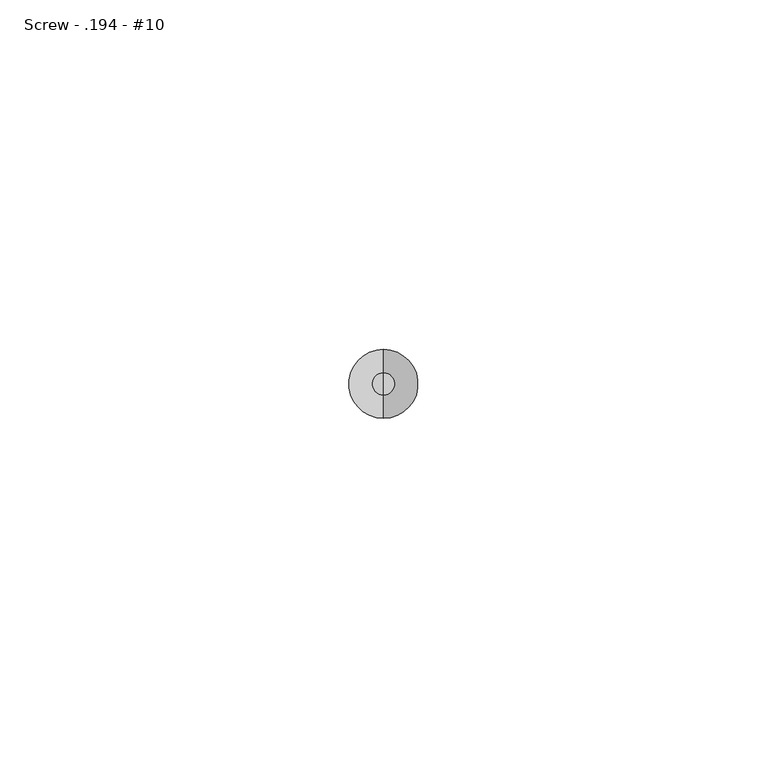
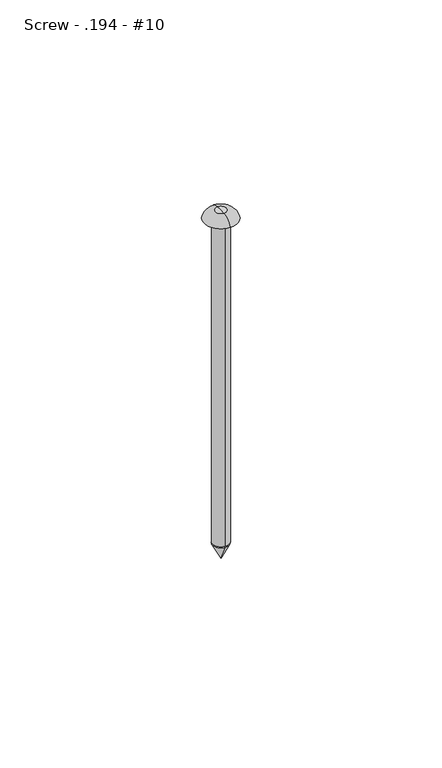
"""IFC4 building model written with IfcOpenShell, lengths in millimetres: fastener geometry, 060523 - W_P_C - Fastenings - Generic : Screw - .194 - #10."""

import ifcopenshell
import ifcopenshell.guid

model = None  # the IFC model being written
_history = None  # IfcOwnerHistory: only IFC2X3 demands one
_inside = {}  # id of a spatial element -> (the spatial element, [elements in it])
_under = {}  # id of a project, library or spatial element -> (it, [spatial elements below it])
_declared = {}  # id of a project -> (the project, [libraries it declares])
_typed = {}  # id of a type object -> (the type object, [elements of that type])
_made_of = {}  # id of a material, layer set ... -> (it, [elements and type objects made of it])


def new_model(schema):
    """Start an empty IFC model of exactly this schema.

    Asked for "IFC4X3", IfcOpenShell would pick the latest addendum, in which some entities
    have other attributes; the version numbers below select the first issue.
    IFC2X3 requires an IfcOwnerHistory on every rooted entity: one is made here for all.
    """
    global model, _history
    if schema == "IFC4X3":
        model = ifcopenshell.file(schema_version=(4, 3, 0, 0))
    else:
        model = ifcopenshell.file(schema=schema)
    _inside.clear()
    _under.clear()
    _declared.clear()
    _typed.clear()
    _made_of.clear()
    _history = None
    if model.schema == "IFC2X3":
        org = make("IfcOrganization", Name="unknown")
        user = make(
            "IfcPersonAndOrganization",
            ThePerson=make("IfcPerson", FamilyName="unknown"),
            TheOrganization=org,
        )
        app = make(
            "IfcApplication",
            ApplicationDeveloper=org,
            Version="unknown",
            ApplicationFullName="unknown",
            ApplicationIdentifier="unknown",
        )
        _history = make(
            "IfcOwnerHistory",
            OwningUser=user,
            OwningApplication=app,
            ChangeAction="ADDED",
            CreationDate=0,
        )
    return model


def make(cls, **values):
    """One entity of the class cls with the attributes given. An attribute that is None is left unset."""
    return model.create_entity(
        cls, **{name: value for name, value in values.items() if value is not None}
    )


def rooted(cls, **values):
    """An entity with a GlobalId (a new one), such as an element, a storey or a relation."""
    return make(cls, GlobalId=ifcopenshell.guid.new(), OwnerHistory=_history, **values)


def si_unit(unit_type, name, prefix=None):
    """IfcSIUnit, for example si_unit("LENGTHUNIT", "METRE", prefix="MILLI")."""
    return make("IfcSIUnit", UnitType=unit_type, Prefix=prefix, Name=name)


def assignment(units):
    """IfcUnitAssignment: the units of a project."""
    return None if units is None else make("IfcUnitAssignment", Units=units)


def point(xyz):
    """IfcCartesianPoint."""
    return None if xyz is None else make("IfcCartesianPoint", Coordinates=xyz)


def direction(xyz):
    """IfcDirection."""
    return None if xyz is None else make("IfcDirection", DirectionRatios=xyz)


def frame(location, z_axis=None, x_axis=None):
    """IfcAxis2Placement3D, a coordinate frame: its origin and axes. An axis left out is left unset."""
    return make(
        "IfcAxis2Placement3D",
        Location=point(location),
        Axis=direction(z_axis),
        RefDirection=direction(x_axis),
    )


def frame_2d(location, x_axis=None):
    """IfcAxis2Placement2D, a coordinate frame in the plane: its origin and x axis."""
    return make(
        "IfcAxis2Placement2D", Location=point(location), RefDirection=direction(x_axis)
    )


def origin():
    """The frame at (0, 0, 0) with its axes left unset."""
    return frame((0.0, 0.0, 0.0))


def origin_2d():
    """The frame at (0, 0) in the plane with its x axis left unset."""
    return frame_2d((0.0, 0.0))


def place(relative_to, where):
    """IfcLocalPlacement: puts the frame where relative to a parent placement (None: the world)."""
    return make(
        "IfcLocalPlacement", PlacementRelTo=relative_to, RelativePlacement=where
    )


def context(
    kind, dimensions, precision=None, world=None, true_north=None, identifier=None
):
    """IfcGeometricRepresentationContext, for example the 3D "Model" context."""
    return make(
        "IfcGeometricRepresentationContext",
        ContextIdentifier=identifier,
        ContextType=kind,
        CoordinateSpaceDimension=dimensions,
        Precision=precision,
        WorldCoordinateSystem=world,
        TrueNorth=true_north,
    )


def project(units=None, contexts=None):
    """IfcProject with its units and contexts."""
    return rooted(
        "IfcProject",
        Name="project",
        RepresentationContexts=contexts,
        UnitsInContext=assignment(units),
    )


def spatial(cls, under=None, at=None, **own):
    """A site, building, storey or space (cls), placed at a placement, below another one or the project."""
    s = rooted(cls, ObjectPlacement=at, **own)
    if under is not None:
        _under.setdefault(under.id(), (under, []))[1].append(s)
    return s


def polyline(points):
    """IfcPolyline through the points."""
    return make("IfcPolyline", Points=[point(p) for p in points])


def circle_curve(where, radius):
    """IfcCircle in the frame where."""
    return make("IfcCircle", Position=where, Radius=radius)


def ellipse_curve(where, semi_axis1, semi_axis2):
    """IfcEllipse in the frame where."""
    return make(
        "IfcEllipse", Position=where, SemiAxis1=semi_axis1, SemiAxis2=semi_axis2
    )


def trimmed(basis, trim1, trim2, sense, master):
    """IfcTrimmedCurve: the piece of a basis curve between two trims."""
    return make(
        "IfcTrimmedCurve",
        BasisCurve=basis,
        Trim1=trim1,
        Trim2=trim2,
        SenseAgreement=sense,
        MasterRepresentation=master,
    )


def segment(curve, same_sense, transition):
    """IfcCompositeCurveSegment."""
    return make(
        "IfcCompositeCurveSegment",
        Transition=transition,
        SameSense=same_sense,
        ParentCurve=curve,
    )


def composite_curve(segments, self_intersect=None):
    """IfcCompositeCurve: segments joined end to end."""
    return make("IfcCompositeCurve", Segments=segments, SelfIntersect=self_intersect)


def outline(outer, holes=None, kind="AREA"):
    """IfcArbitraryClosedProfileDef: a profile drawn as a closed curve; with holes, ...WithVoids."""
    if holes is None:
        return make("IfcArbitraryClosedProfileDef", ProfileType=kind, OuterCurve=outer)
    return make(
        "IfcArbitraryProfileDefWithVoids",
        ProfileType=kind,
        OuterCurve=outer,
        InnerCurves=holes,
    )


def extrude(swept, where, along, depth):
    """IfcExtrudedAreaSolid: the profile swept, set in the frame where, extruded along a direction by depth."""
    return make(
        "IfcExtrudedAreaSolid",
        SweptArea=swept,
        Position=where,
        ExtrudedDirection=direction(along),
        Depth=depth,
    )


def shape(context_of_items, identifier, shape_type, items):
    """IfcShapeRepresentation: the items that make up one representation, for example the "Body"."""
    return make(
        "IfcShapeRepresentation",
        ContextOfItems=context_of_items,
        RepresentationIdentifier=identifier,
        RepresentationType=shape_type,
        Items=items,
    )


def source(mapping_origin, context_of_items, identifier, shape_type, items):
    """IfcRepresentationMap: a shape defined once, which mapped items show again and again."""
    return make(
        "IfcRepresentationMap",
        MappingOrigin=mapping_origin,
        MappedRepresentation=shape(context_of_items, identifier, shape_type, items),
    )


def transform(
    local_origin,
    x_axis=None,
    y_axis=None,
    z_axis=None,
    scale=None,
    scale2=None,
    scale3=None,
    uniform=True,
):
    """IfcCartesianTransformationOperator3D, or its non-uniform kind. x_axis, y_axis, z_axis: its Axis1, 2, 3."""
    if uniform:
        return make(
            "IfcCartesianTransformationOperator3D",
            Axis1=direction(x_axis),
            Axis2=direction(y_axis),
            LocalOrigin=point(local_origin),
            Scale=scale,
            Axis3=direction(z_axis),
        )
    return make(
        "IfcCartesianTransformationOperator3DnonUniform",
        Axis1=direction(x_axis),
        Axis2=direction(y_axis),
        LocalOrigin=point(local_origin),
        Scale=scale,
        Axis3=direction(z_axis),
        Scale2=scale2,
        Scale3=scale3,
    )


def mapped(mapping_source, mapping_target):
    """IfcMappedItem: shows the shape of a source again, moved by a transform."""
    return make(
        "IfcMappedItem", MappingSource=mapping_source, MappingTarget=mapping_target
    )


def made_of(thing, what):
    """Note that an element or type object is made of a material, layer set ...; save() writes the relation."""
    if what is not None:
        _made_of.setdefault(what.id(), (what, []))[1].append(thing)
    return thing


def element(
    cls,
    number,
    at=None,
    inside=None,
    cuts=None,
    type_object=None,
    material=None,
    context=None,
    identifier="Body",
    shape_type=None,
    held_by="IfcProductDefinitionShape",
    body=None,
    shapes=None,
    **own,
):
    """One element of the class cls, such as IfcWall. Its Tag is "e" and its number.

    at: its placement. inside: the storey or other place that contains it. cuts: it is an
    opening in that element (IfcRelVoidsElement). A single representation is given by context,
    identifier, shape_type and body (its items); several are given by shapes. held_by: the class
    of the entity that holds the representations. save() writes the other relations.
    """
    e = rooted(cls, Tag="e%d" % number, ObjectPlacement=at, **own)
    if body is not None:
        shapes = [shape(context, identifier, shape_type, body)]
    if shapes is not None:
        e.Representation = make(held_by, Representations=shapes)
    if inside is not None:
        _inside.setdefault(inside.id(), (inside, []))[1].append(e)
    if cuts is not None:
        rooted(
            "IfcRelVoidsElement", RelatingBuildingElement=cuts, RelatedOpeningElement=e
        )
    if type_object is not None:
        _typed.setdefault(type_object.id(), (type_object, []))[1].append(e)
    return made_of(e, material)


def aggregate(whole, parts):
    """IfcRelAggregates: a whole, such as a stair, and the parts it consists of."""
    return rooted("IfcRelAggregates", RelatingObject=whole, RelatedObjects=parts)


def save(model, path):
    """Write the relations noted so far, then the file.

    IfcRelAggregates (storeys below a building ...), IfcRelContainedInSpatialStructure (elements
    in a storey), IfcRelDefinesByType, IfcRelAssociatesMaterial and IfcRelDeclares: one each for
    every whole, place, type object, material and project.
    """
    for whole, parts in _under.values():
        aggregate(whole, parts)
    for where, things in _inside.values():
        rooted(
            "IfcRelContainedInSpatialStructure",
            RelatedElements=things,
            RelatingStructure=where,
        )
    for kind, things in _typed.values():
        rooted("IfcRelDefinesByType", RelatedObjects=things, RelatingType=kind)
    for what, things in _made_of.values():
        rooted("IfcRelAssociatesMaterial", RelatedObjects=things, RelatingMaterial=what)
    for by, libraries in _declared.values():
        rooted("IfcRelDeclares", RelatingContext=by, RelatedDefinitions=libraries)
    model.write(path)


def plane_surface(at):
    """IfcPlane: the flat surface through the origin of the frame at, square to its z axis."""
    return make("IfcPlane", Position=at)


def revolved_surface(curve, axis_point, axis_direction):
    """IfcSurfaceOfRevolution: the curve turned about the line through axis_point along axis_direction."""
    return make(
        "IfcSurfaceOfRevolution",
        SweptCurve=make("IfcArbitraryOpenProfileDef", ProfileType="CURVE", Curve=curve),
        AxisPosition=make("IfcAxis1Placement", Location=point(axis_point), Axis=direction(axis_direction)),
    )


def advanced_brep(points, edges, surfaces, faces):
    """IfcAdvancedBrep: a solid bounded by faces that lie on surfaces and meet in shared edges.

    An edge is (start, end): straight between two places in points (the first is 0);
    or (start, end, curve); or (start, end, curve, False) where it runs against its curve.
    A face is (place in surfaces, loops), or (place, loops, False) where it looks against
    its surface's normal. A loop lists edges by number (the first is 1), with a minus sign
    where the edge is run from its end to its start. The first loop is the outer one.
    """
    corners = [point(p) for p in points]
    vertices = [make("IfcVertexPoint", VertexGeometry=c) for c in corners]
    made = []
    for start, end, *more in edges:
        made.append(
            make(
                "IfcEdgeCurve",
                EdgeStart=vertices[start],
                EdgeEnd=vertices[end],
                EdgeGeometry=more[0] if more else make("IfcPolyline", Points=[corners[start], corners[end]]),
                SameSense=more[1] if len(more) > 1 else True,
            )
        )
    hull = []
    for where, loops, *sense in faces:
        bounds = []
        for j, loop in enumerate(loops):
            ring = [make("IfcOrientedEdge", EdgeElement=made[abs(k) - 1], Orientation=k > 0) for k in loop]
            bounds.append(
                make(
                    "IfcFaceOuterBound" if j == 0 else "IfcFaceBound",
                    Bound=make("IfcEdgeLoop", EdgeList=ring),
                    Orientation=True,
                )
            )
        hull.append(make("IfcAdvancedFace", Bounds=bounds, FaceSurface=surfaces[where], SameSense=sense[0] if sense else True))
    return make("IfcAdvancedBrep", Outer=make("IfcClosedShell", CfsFaces=hull))


def screw_194_10_6687bdcb(model_context):
    return source(origin(), model_context, "Body", "SolidModel", [
        advanced_brep(
        [(0.0, -2.4638, -101.6), (0.0, 2.4638, -101.6), (0.0, 0.0, -101.6), (0.0, 0.0, -106.5276)],
        [
            (0, 1, circle_curve(frame((0.0, 0.0, -101.6), z_axis=(0.0, 0.0, 1.0), x_axis=(0.0, 1.0, 0.0)), 2.4638)),
            (1, 2),
            (2, 0),
            (1, 0, circle_curve(frame((0.0, 0.0, -101.6), z_axis=(0.0, 0.0, 1.0), x_axis=(0.0, 1.0, 0.0)), 2.4638)),
            (3, 1),
            (0, 3),
        ],
        [
            plane_surface(frame((0.0, 0.0, -101.6), z_axis=(0.0, 0.0, 1.0), x_axis=(0.0, 1.0, 0.0))),
            revolved_surface(polyline([(0.0, 2.4638, -101.6), (0.0, 0.0, -106.5276)]), (0.0, 0.0, -103.0840259), (0.0, 0.0, -1.0)),
        ],
        [
            (0, [[1, 2, 3]]),
            (0, [[4, -3, -2]]),
            (1, [[5, -1, 6]]),
            (1, [[-6, -4, -5]]),
        ],
    ),
        advanced_brep(
        [(0.0, 4.9276, 0.0), (0.0, -4.9276, 0.0), (0.0, 0.0, 0.0), (0.0, 0.0, 2.4638), (0.0, -1.5875, 2.4638), (0.0, 1.5875, 2.4638)],
        [
            (0, 1, circle_curve(frame((0.0, 0.0, 0.0), z_axis=(0.0, 0.0, -1.0), x_axis=(0.0, -1.0, 0.0)), 4.9276)),
            (1, 2),
            (2, 0),
            (1, 0, circle_curve(frame((0.0, 0.0, 0.0), z_axis=(0.0, 0.0, -1.0), x_axis=(0.0, -1.0, 0.0)), 4.9276)),
            (3, 4),
            (4, 5, circle_curve(frame((0.0, 0.0, 2.4638), z_axis=(0.0, 0.0, 1.0), x_axis=(0.0, -1.0, 0.0)), 1.5875)),
            (5, 3),
            (5, 4, circle_curve(frame((0.0, 0.0, 2.4638), z_axis=(0.0, 0.0, 1.0), x_axis=(0.0, -1.0, 0.0)), 1.5875)),
            (4, 1, circle_curve(frame((0.0, -1.5875, -1.0321369), z_axis=(1.0, 0.0, 0.0), x_axis=(0.0, -1.0, 0.0)), 3.4959369)),
            (0, 5, circle_curve(frame((0.0, 1.5875, -1.0321369), z_axis=(1.0, 0.0, 0.0), x_axis=(0.0, 1.0, 0.0)), 3.4959369)),
        ],
        [
            plane_surface(frame((0.0, 0.0, 0.0), z_axis=(0.0, 0.0, -1.0), x_axis=(0.0, -1.0, 0.0))),
            plane_surface(frame((0.0, 0.0, 2.4638), z_axis=(0.0, 0.0, 1.0), x_axis=(0.0, -1.0, 0.0))),
            revolved_surface(trimmed(ellipse_curve(frame((0.0, -1.5875, -1.0321369), z_axis=(-1.0, 0.0, 0.0), x_axis=(0.0, -1.0, 0.0)), 3.4959369, 3.4959369), [point((0.0, -4.9276, 0.0))], [point((0.0, -1.5875, 2.4638))], True, "CARTESIAN"), (0.0, 0.0, 1.4840259), (0.0, 0.0, 1.0)),
        ],
        [
            (0, [[1, 2, 3]]),
            (0, [[4, -3, -2]]),
            (1, [[5, 6, 7]]),
            (1, [[-7, 8, -5]]),
            (2, [[-6, 9, -1, 10]]),
            (2, [[-8, -10, -4, -9]]),
        ],
    ),
        extrude(outline(composite_curve([segment(trimmed(circle_curve(origin_2d(), 2.4638), [point((0.0, -2.4638))], [point((0.0, 2.4638))], False, "CARTESIAN"), True, "CONTINUOUS"), segment(trimmed(circle_curve(origin_2d(), 2.4638), [point((0.0, 2.4638))], [point((0.0, -2.4638))], False, "CARTESIAN"), True, "CONTINUOUS")], self_intersect=False)), frame((0.0, 0.0, -101.6), z_axis=(0.0, 0.0, 1.0), x_axis=(1.0, 0.0, 0.0)), (0.0, 0.0, 1.0), 101.6),
    ])


if __name__ == "__main__":
    model = new_model("IFC4")
    model_context = context("Model", 3, world=origin())
    ifc_project = project(units=[si_unit("LENGTHUNIT", "METRE", prefix="MILLI")], contexts=[model_context])
    site = spatial("IfcSite", under=ifc_project)
    building = spatial("IfcBuilding", under=site)
    placement = place(None, origin())
    screw_194_10_shape = screw_194_10_6687bdcb(model_context)
    element("IfcFastener", 1, ObjectType="060523 - W_P_C - Fastenings - Generic : Screw - .194 - #10", at=placement, inside=building, context=model_context, shape_type="MappedRepresentation", body=[
        mapped(screw_194_10_shape, transform((0.0, 0.0, 0.0), x_axis=(1.0, 0.0, 0.0), y_axis=(0.0, 1.0, 0.0), z_axis=(0.0, 0.0, 1.0))),
    ])
    save(model, "model.ifc")

# Revit data of these elements
# Type "060523 - W_P_C - Fastenings - Generic : Screw - .194 - #10"
#   Washer_Thickness = 0' - 0.00333"
#   Washer Radius = 0' - 0.107"
#   Washer Offset - Head = 0' - 0"
#   Washer Offset = 0' - 0"
#   Thickness_of_Substrate [instance default] = 0' - 1"
#   Side = 0' - 0 37/64"
#   Radius = 0' - 0.097"
#   Length [instance default] = 0' - 4"
#   Head Size = 0' - 1"
#   Head Radius = 0' - 0 1/2"
#   Head Height = 0' - 0.01"
#   Double Diameter = 0' - 0.388"
#   Diameter = 0' - 0.194"
#   Default Elevation = 4' - 0"
#   Washer_Nut_Visibility = no
#   Washer_Head_Visibility = no
#   Round_Head_Visibility = yes
#   Point Visibility = yes
#   Nut_Visibility = no
#   Hex_Head_Visiblilty = no
#   Washer Material = none
#   Bolt Material (Size) = AT SILL - FASTENER AT 24" O.C.
# Element 1 (IfcFastener, "060523 - W_P_C - Fastenings - Generic : Screw - .194 - #10")
#   Materials on its faces: "AT SILL - FASTENER AT 24\" O.C."
# Materials
#   "AT SILL - FASTENER AT 24\" O.C.": class "Generic", colour RGB 120 120 120, transparency 0, Cost = 0
